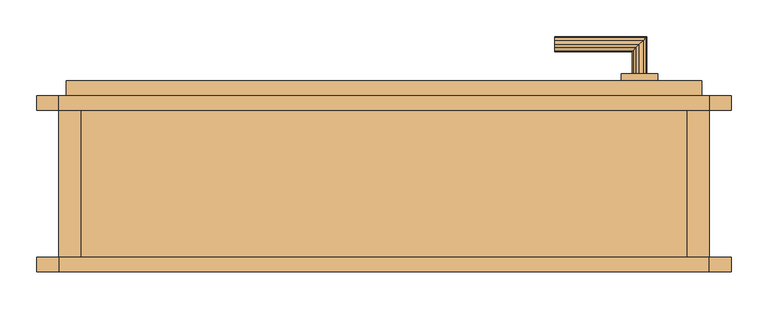
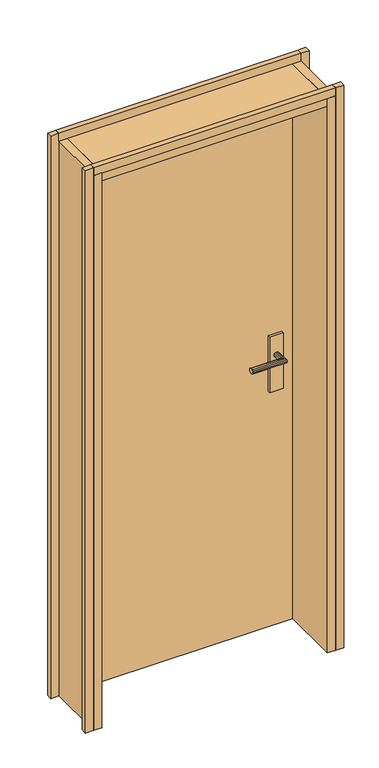
"""IFC4 building model written with IfcOpenShell, lengths in millimetres: door geometry, Tür."""

from ifc_helpers import new_model, si_unit, frame, origin, place, context, project, spatial, polyline, outline, extrude, faceted_brep, source, transform, mapped, element, save


def door_d8db362f(model_context):
    return source(origin(), model_context, "Body", "SolidModel", [
        extrude(outline(polyline([(915.0, 0.0), (915.0, -20.0), (885.0, -20.0), (885.0, 0.0), (915.0, 0.0)])), frame((0.0, 0.0, 140.0), z_axis=(0.0, 0.0, 1.0), x_axis=(1.0, 0.0, 0.0)), (0.0, 0.0, 1.0), 2175.0),
        extrude(outline(polyline([(885.0, 220.0), (885.0, 200.0), (0.0, 200.0), (0.0, 220.0), (885.0, 220.0)])), frame((0.0, 0.0, 2285.0), z_axis=(0.0, 0.0, 1.0), x_axis=(1.0, 0.0, 0.0)), (0.0, 0.0, 1.0), 30.0),
        extrude(outline(polyline([(765.0, 200.0), (815.0, 200.0), (815.0, 190.0), (765.0, 190.0), (765.0, 200.0)])), frame((0.0, 0.0, 1050.0), z_axis=(0.0, 0.0, 1.0), x_axis=(1.0, 0.0, 0.0)), (0.0, 0.0, 1.0), 215.0),
        extrude(outline(polyline([(0.0, -20.0), (-30.0, -20.0), (-30.0, 0.0), (0.0, 0.0), (0.0, -20.0)])), frame((0.0, 0.0, 140.0), z_axis=(0.0, 0.0, 1.0), x_axis=(1.0, 0.0, 0.0)), (0.0, 0.0, 1.0), 2175.0),
        extrude(outline(polyline([(915.0, 220.0), (915.0, 200.0), (885.0, 200.0), (885.0, 220.0), (915.0, 220.0)])), frame((0.0, 0.0, 140.0), z_axis=(0.0, 0.0, 1.0), x_axis=(1.0, 0.0, 0.0)), (0.0, 0.0, 1.0), 2175.0),
        extrude(outline(polyline([(30.0, 220.0), (30.0, -20.0), (0.0, -20.0), (0.0, 220.0), (30.0, 220.0)])), frame((0.0, 0.0, 140.0), z_axis=(0.0, 0.0, 1.0), x_axis=(1.0, 0.0, 0.0)), (0.0, 0.0, 1.0), 2145.0),
        extrude(outline(polyline([(875.0, 240.0), (875.0, 200.0), (10.0, 200.0), (10.0, 240.0), (875.0, 240.0)])), frame((0.0, 0.0, 140.0), z_axis=(0.0, 0.0, 1.0), x_axis=(1.0, 0.0, 0.0)), (0.0, 0.0, 1.0), 2135.0),
        extrude(outline(polyline([(885.0, 0.0), (885.0, -20.0), (0.0, -20.0), (0.0, 0.0), (885.0, 0.0)])), frame((0.0, 0.0, 2285.0), z_axis=(0.0, 0.0, 1.0), x_axis=(1.0, 0.0, 0.0)), (0.0, 0.0, 1.0), 30.0),
        extrude(outline(polyline([(0.0, 200.0), (-30.0, 200.0), (-30.0, 220.0), (0.0, 220.0), (0.0, 200.0)])), frame((0.0, 0.0, 140.0), z_axis=(0.0, 0.0, 1.0), x_axis=(1.0, 0.0, 0.0)), (0.0, 0.0, 1.0), 2175.0),
        extrude(outline(polyline([(885.0, 220.0), (885.0, -20.0), (855.0, -20.0), (855.0, 220.0), (885.0, 220.0)])), frame((0.0, 0.0, 140.0), z_axis=(0.0, 0.0, 1.0), x_axis=(1.0, 0.0, 0.0)), (0.0, 0.0, 1.0), 2145.0),
        extrude(outline(polyline([(815.0, 250.0), (815.0, 240.0), (765.0, 240.0), (765.0, 250.0), (815.0, 250.0)])), frame((0.0, 0.0, 1050.0), z_axis=(0.0, 0.0, 1.0), x_axis=(1.0, 0.0, 0.0)), (0.0, 0.0, 1.0), 215.0),
        faceted_brep([(795.0, 250.0, 1198.660254), (790.0, 250.0, 1200.0), (785.0, 250.0, 1198.660254), (781.339746, 250.0, 1195.0), (780.0, 250.0, 1190.0), (781.339746, 250.0, 1185.0), (785.0, 250.0, 1181.339746), (790.0, 250.0, 1180.0), (795.0, 250.0, 1181.339746), (798.660254, 250.0, 1185.0), (800.0, 250.0, 1190.0), (798.660254, 250.0, 1195.0), (790.0, 290.0, 1200.0), (795.0, 295.0, 1198.660254), (798.660254, 298.660254, 1195.0), (800.0, 300.0, 1190.0), (798.660254, 298.660254, 1185.0), (795.0, 295.0, 1181.339746), (790.0, 290.0, 1180.0), (785.0, 285.0, 1181.339746), (781.339746, 281.339746, 1185.0), (780.0, 280.0, 1190.0), (781.339746, 281.339746, 1195.0), (785.0, 285.0, 1198.660254), (675.0, 285.0, 1198.660254), (675.0, 290.0, 1200.0), (675.0, 295.0, 1198.660254), (675.0, 298.660254, 1195.0), (675.0, 300.0, 1190.0), (675.0, 298.660254, 1185.0), (675.0, 295.0, 1181.339746), (675.0, 290.0, 1180.0), (675.0, 285.0, 1181.339746), (675.0, 281.339746, 1185.0), (675.0, 280.0, 1190.0), (675.0, 281.339746, 1195.0)], [[[0, 1, 2, 3, 4, 5, 6, 7, 8, 9, 10, 11]], [[12, 1, 0, 13]], [[13, 0, 11, 14]], [[14, 11, 10, 15]], [[15, 10, 9, 16]], [[16, 9, 8, 17]], [[17, 8, 7, 18]], [[18, 7, 6, 19]], [[19, 6, 5, 20]], [[20, 5, 4, 21]], [[21, 4, 3, 22]], [[22, 3, 2, 23]], [[23, 2, 1, 12]], [[24, 25, 26, 27, 28, 29, 30, 31, 32, 33, 34, 35]], [[25, 12, 13, 26]], [[26, 13, 14, 27]], [[27, 14, 15, 28]], [[28, 15, 16, 29]], [[29, 16, 17, 30]], [[30, 17, 18, 31]], [[31, 18, 19, 32]], [[32, 19, 20, 33]], [[33, 20, 21, 34]], [[34, 21, 22, 35]], [[35, 22, 23, 24]], [[24, 23, 12, 25]]]),
        extrude(outline(polyline([(855.0, 220.0), (855.0, -20.0), (30.0, -20.0), (30.0, 220.0), (855.0, 220.0)])), frame((0.0, 0.0, 2255.0), z_axis=(0.0, 0.0, 1.0), x_axis=(1.0, 0.0, 0.0)), (0.0, 0.0, 1.0), 30.0),
        faceted_brep([(785.0, 190.0, 1198.660254), (790.0, 190.0, 1200.0), (795.0, 190.0, 1198.660254), (798.660254, 190.0, 1195.0), (800.0, 190.0, 1190.0), (798.660254, 190.0, 1185.0), (795.0, 190.0, 1181.339746), (790.0, 190.0, 1180.0), (785.0, 190.0, 1181.339746), (781.339746, 190.0, 1185.0), (780.0, 190.0, 1190.0), (781.339746, 190.0, 1195.0), (790.0, 150.0, 1200.0), (795.0, 145.0, 1198.660254), (798.660254, 141.339746, 1195.0), (800.0, 140.0, 1190.0), (798.660254, 141.339746, 1185.0), (795.0, 145.0, 1181.339746), (790.0, 150.0, 1180.0), (785.0, 155.0, 1181.339746), (781.339746, 158.660254, 1185.0), (780.0, 160.0, 1190.0), (781.339746, 158.660254, 1195.0), (785.0, 155.0, 1198.660254), (675.0, 145.0, 1198.660254), (675.0, 150.0, 1200.0), (675.0, 155.0, 1198.660254), (675.0, 158.660254, 1195.0), (675.0, 160.0, 1190.0), (675.0, 158.660254, 1185.0), (675.0, 155.0, 1181.339746), (675.0, 150.0, 1180.0), (675.0, 145.0, 1181.339746), (675.0, 141.339746, 1185.0), (675.0, 140.0, 1190.0), (675.0, 141.339746, 1195.0)], [[[0, 1, 2, 3, 4, 5, 6, 7, 8, 9, 10, 11]], [[2, 1, 12, 13]], [[3, 2, 13, 14]], [[4, 3, 14, 15]], [[5, 4, 15, 16]], [[6, 5, 16, 17]], [[7, 6, 17, 18]], [[8, 7, 18, 19]], [[9, 8, 19, 20]], [[10, 9, 20, 21]], [[11, 10, 21, 22]], [[0, 11, 22, 23]], [[1, 0, 23, 12]], [[24, 25, 26, 27, 28, 29, 30, 31, 32, 33, 34, 35]], [[13, 12, 25, 24]], [[14, 13, 24, 35]], [[15, 14, 35, 34]], [[16, 15, 34, 33]], [[17, 16, 33, 32]], [[18, 17, 32, 31]], [[19, 18, 31, 30]], [[20, 19, 30, 29]], [[21, 20, 29, 28]], [[22, 21, 28, 27]], [[23, 22, 27, 26]], [[12, 23, 26, 25]]]),
    ])


if __name__ == "__main__":
    model = new_model("IFC4")
    model_context = context("Model", 3, world=origin())
    ifc_project = project(units=[si_unit("LENGTHUNIT", "METRE", prefix="MILLI")], contexts=[model_context])
    site = spatial("IfcSite", under=ifc_project)
    building = spatial("IfcBuilding", under=site)
    placement = place(None, origin())
    door_shape = door_d8db362f(model_context)
    element("IfcDoor", 1, ObjectType="Tür", at=placement, inside=building, context=model_context, shape_type="MappedRepresentation", body=[
        mapped(door_shape, transform((0.0, 0.0, 0.0), x_axis=(1.0, 0.0, 0.0), y_axis=(0.0, 1.0, 0.0), z_axis=(0.0, 0.0, 1.0))),
    ])
    save(model, "model.ifc")

# Revit data of these elements
# Type "Tür"
#   Type Mark = "35"
# Element 1 (IfcDoor, "Tür")
#   Materials on its faces: "tuer_beschlag", "tuer_holzzarge"
# Materials
#   "tuer_beschlag": class "Unassigned", colour RGB 128 128 128, transparency 0
#   "tuer_holzzarge": class "Unassigned", colour RGB 255 255 255, transparency 0
